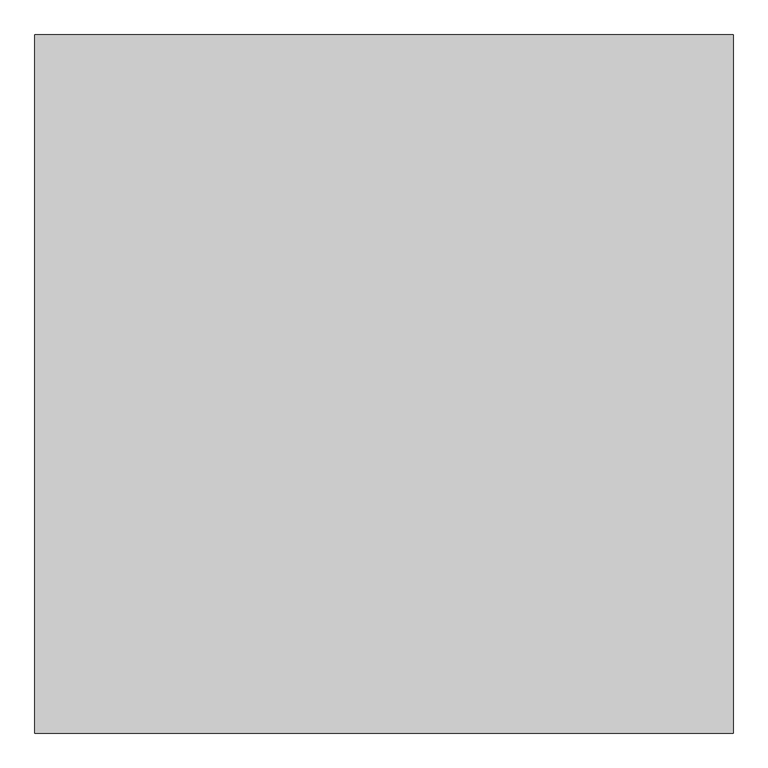
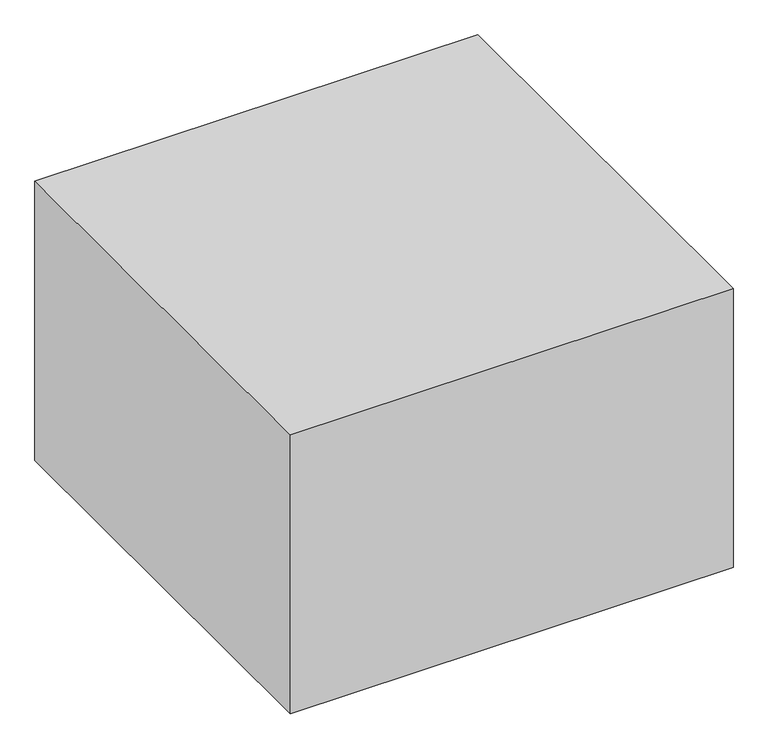
"""IFC4 building model written with IfcOpenShell, lengths in millimetres: proxy geometry, Space Planning Box_hec : Space Planning Box_hec."""

from ifc_helpers import new_model, si_unit, origin, origin_with_axes, place, context, project, spatial, polyline, outline, extrude, source, transform, mapped, element, save


def generic_models_b79df083(model_context):
    return source(origin(), model_context, "Body", "SweptSolid", [
        extrude(outline(polyline([(4500.0, 4500.0), (4500.0, -4500.0), (-4500.0, -4500.0), (-4500.0, 4500.0), (4500.0, 4500.0)])), origin_with_axes(), (0.0, 0.0, 1.0), 6000.0),
    ])


if __name__ == "__main__":
    model = new_model("IFC4")
    model_context = context("Model", 3, world=origin())
    ifc_project = project(units=[si_unit("LENGTHUNIT", "METRE", prefix="MILLI")], contexts=[model_context])
    site = spatial("IfcSite", under=ifc_project)
    building = spatial("IfcBuilding", under=site)
    placement = place(None, origin())
    generic_models_shape = generic_models_b79df083(model_context)
    element("IfcBuildingElementProxy", 1, Name="Space Planning Box_hec : Space Planning Box_hec", ObjectType="Space Planning Box_hec : Space Planning Box_hec", at=placement, inside=building, context=model_context, shape_type="MappedRepresentation", body=[
        mapped(generic_models_shape, transform((0.0, 0.0, 0.0), x_axis=(1.0, 0.0, 0.0), y_axis=(0.0, 1.0, 0.0), z_axis=(0.0, 0.0, 1.0))),
    ])
    save(model, "model.ifc")

# Revit data of these elements
# Type "Space Planning Box_hec : Space Planning Box_hec"
#   Type Comments = "..."
#   Room Name [instance default] = "?"
#   Interior Finish [instance default] = ""
#   Exterior Finish [instance default] = ""
#   Department [instance default] = ""
#   Assembly Code = "..."
#   Width [instance default] = 1524 mm
#   Program Area [instance default] = 0 m²
#   Length [instance default] = 1524 mm
#   Height [instance default] = 1524 mm
#   Area [instance default] = 2.32258 m²
#   Fill Color [instance default] = Cyan
#   Default Elevation = 0
# Element 1 (IfcBuildingElementProxy, "Space Planning Box_hec : Space Planning Box_hec")
#   Room Name = "Kitch & Lunch Room"
#   Interior Finish = "IF2-1"
#   Exterior Finish = "EF1"
#   Department = "AR"
#   Width = 9000 mm
#   Program Area = 31.5 m²
#   Length = 9000 mm
#   Height = 6000 mm
#   Area = 81 m²
#   Fill Color = Lavender
#   Materials on its faces: "Lavender"
# Materials
#   "Cyan": class "Generic", colour RGB 0 255 255, transparency 0.2, Cost = 0
#   "Lavender": class "Generic", colour RGB 186 85 211, transparency 0.2, Cost = 0
